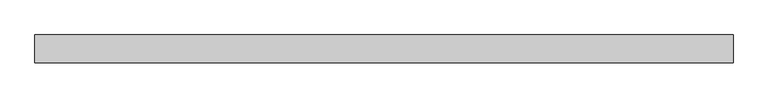
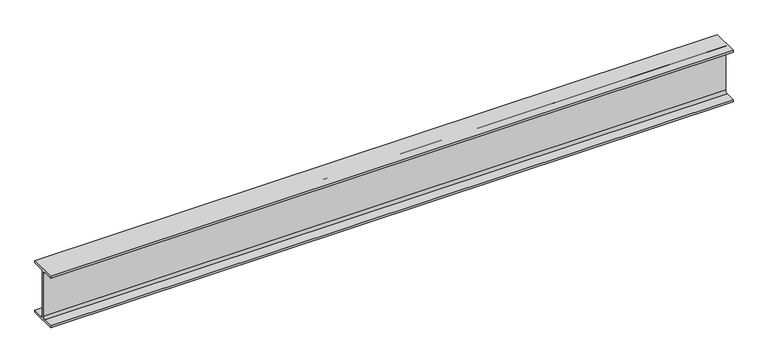
"""IFC4 building model written with IfcOpenShell, lengths in millimetres: beam geometry, 0912_Steel Framing_H-KSD3502 : H_SB_ASB_H-250x125x6x9."""

import ifcopenshell
import ifcopenshell.guid

model = None  # the IFC model being written
_history = None  # IfcOwnerHistory: only IFC2X3 demands one
_inside = {}  # id of a spatial element -> (the spatial element, [elements in it])
_under = {}  # id of a project, library or spatial element -> (it, [spatial elements below it])
_declared = {}  # id of a project -> (the project, [libraries it declares])
_typed = {}  # id of a type object -> (the type object, [elements of that type])
_made_of = {}  # id of a material, layer set ... -> (it, [elements and type objects made of it])


def new_model(schema):
    """Start an empty IFC model of exactly this schema.

    Asked for "IFC4X3", IfcOpenShell would pick the latest addendum, in which some entities
    have other attributes; the version numbers below select the first issue.
    IFC2X3 requires an IfcOwnerHistory on every rooted entity: one is made here for all.
    """
    global model, _history
    if schema == "IFC4X3":
        model = ifcopenshell.file(schema_version=(4, 3, 0, 0))
    else:
        model = ifcopenshell.file(schema=schema)
    _inside.clear()
    _under.clear()
    _declared.clear()
    _typed.clear()
    _made_of.clear()
    _history = None
    if model.schema == "IFC2X3":
        org = make("IfcOrganization", Name="unknown")
        user = make(
            "IfcPersonAndOrganization",
            ThePerson=make("IfcPerson", FamilyName="unknown"),
            TheOrganization=org,
        )
        app = make(
            "IfcApplication",
            ApplicationDeveloper=org,
            Version="unknown",
            ApplicationFullName="unknown",
            ApplicationIdentifier="unknown",
        )
        _history = make(
            "IfcOwnerHistory",
            OwningUser=user,
            OwningApplication=app,
            ChangeAction="ADDED",
            CreationDate=0,
        )
    return model


def make(cls, **values):
    """One entity of the class cls with the attributes given. An attribute that is None is left unset."""
    return model.create_entity(
        cls, **{name: value for name, value in values.items() if value is not None}
    )


def rooted(cls, **values):
    """An entity with a GlobalId (a new one), such as an element, a storey or a relation."""
    return make(cls, GlobalId=ifcopenshell.guid.new(), OwnerHistory=_history, **values)


def si_unit(unit_type, name, prefix=None):
    """IfcSIUnit, for example si_unit("LENGTHUNIT", "METRE", prefix="MILLI")."""
    return make("IfcSIUnit", UnitType=unit_type, Prefix=prefix, Name=name)


def assignment(units):
    """IfcUnitAssignment: the units of a project."""
    return None if units is None else make("IfcUnitAssignment", Units=units)


def point(xyz):
    """IfcCartesianPoint."""
    return None if xyz is None else make("IfcCartesianPoint", Coordinates=xyz)


def direction(xyz):
    """IfcDirection."""
    return None if xyz is None else make("IfcDirection", DirectionRatios=xyz)


def frame(location, z_axis=None, x_axis=None):
    """IfcAxis2Placement3D, a coordinate frame: its origin and axes. An axis left out is left unset."""
    return make(
        "IfcAxis2Placement3D",
        Location=point(location),
        Axis=direction(z_axis),
        RefDirection=direction(x_axis),
    )


def frame_2d(location, x_axis=None):
    """IfcAxis2Placement2D, a coordinate frame in the plane: its origin and x axis."""
    return make(
        "IfcAxis2Placement2D", Location=point(location), RefDirection=direction(x_axis)
    )


def origin():
    """The frame at (0, 0, 0) with its axes left unset."""
    return frame((0.0, 0.0, 0.0))


def place(relative_to, where):
    """IfcLocalPlacement: puts the frame where relative to a parent placement (None: the world)."""
    return make(
        "IfcLocalPlacement", PlacementRelTo=relative_to, RelativePlacement=where
    )


def context(
    kind, dimensions, precision=None, world=None, true_north=None, identifier=None
):
    """IfcGeometricRepresentationContext, for example the 3D "Model" context."""
    return make(
        "IfcGeometricRepresentationContext",
        ContextIdentifier=identifier,
        ContextType=kind,
        CoordinateSpaceDimension=dimensions,
        Precision=precision,
        WorldCoordinateSystem=world,
        TrueNorth=true_north,
    )


def project(units=None, contexts=None):
    """IfcProject with its units and contexts."""
    return rooted(
        "IfcProject",
        Name="project",
        RepresentationContexts=contexts,
        UnitsInContext=assignment(units),
    )


def spatial(cls, under=None, at=None, **own):
    """A site, building, storey or space (cls), placed at a placement, below another one or the project."""
    s = rooted(cls, ObjectPlacement=at, **own)
    if under is not None:
        _under.setdefault(under.id(), (under, []))[1].append(s)
    return s


def polyline(points):
    """IfcPolyline through the points."""
    return make("IfcPolyline", Points=[point(p) for p in points])


def circle_curve(where, radius):
    """IfcCircle in the frame where."""
    return make("IfcCircle", Position=where, Radius=radius)


def trimmed(basis, trim1, trim2, sense, master):
    """IfcTrimmedCurve: the piece of a basis curve between two trims."""
    return make(
        "IfcTrimmedCurve",
        BasisCurve=basis,
        Trim1=trim1,
        Trim2=trim2,
        SenseAgreement=sense,
        MasterRepresentation=master,
    )


def segment(curve, same_sense, transition):
    """IfcCompositeCurveSegment."""
    return make(
        "IfcCompositeCurveSegment",
        Transition=transition,
        SameSense=same_sense,
        ParentCurve=curve,
    )


def composite_curve(segments, self_intersect=None):
    """IfcCompositeCurve: segments joined end to end."""
    return make("IfcCompositeCurve", Segments=segments, SelfIntersect=self_intersect)


def outline(outer, holes=None, kind="AREA"):
    """IfcArbitraryClosedProfileDef: a profile drawn as a closed curve; with holes, ...WithVoids."""
    if holes is None:
        return make("IfcArbitraryClosedProfileDef", ProfileType=kind, OuterCurve=outer)
    return make(
        "IfcArbitraryProfileDefWithVoids",
        ProfileType=kind,
        OuterCurve=outer,
        InnerCurves=holes,
    )


def extrude(swept, where, along, depth):
    """IfcExtrudedAreaSolid: the profile swept, set in the frame where, extruded along a direction by depth."""
    return make(
        "IfcExtrudedAreaSolid",
        SweptArea=swept,
        Position=where,
        ExtrudedDirection=direction(along),
        Depth=depth,
    )


def shape(context_of_items, identifier, shape_type, items):
    """IfcShapeRepresentation: the items that make up one representation, for example the "Body"."""
    return make(
        "IfcShapeRepresentation",
        ContextOfItems=context_of_items,
        RepresentationIdentifier=identifier,
        RepresentationType=shape_type,
        Items=items,
    )


def source(mapping_origin, context_of_items, identifier, shape_type, items):
    """IfcRepresentationMap: a shape defined once, which mapped items show again and again."""
    return make(
        "IfcRepresentationMap",
        MappingOrigin=mapping_origin,
        MappedRepresentation=shape(context_of_items, identifier, shape_type, items),
    )


def transform(
    local_origin,
    x_axis=None,
    y_axis=None,
    z_axis=None,
    scale=None,
    scale2=None,
    scale3=None,
    uniform=True,
):
    """IfcCartesianTransformationOperator3D, or its non-uniform kind. x_axis, y_axis, z_axis: its Axis1, 2, 3."""
    if uniform:
        return make(
            "IfcCartesianTransformationOperator3D",
            Axis1=direction(x_axis),
            Axis2=direction(y_axis),
            LocalOrigin=point(local_origin),
            Scale=scale,
            Axis3=direction(z_axis),
        )
    return make(
        "IfcCartesianTransformationOperator3DnonUniform",
        Axis1=direction(x_axis),
        Axis2=direction(y_axis),
        LocalOrigin=point(local_origin),
        Scale=scale,
        Axis3=direction(z_axis),
        Scale2=scale2,
        Scale3=scale3,
    )


def mapped(mapping_source, mapping_target):
    """IfcMappedItem: shows the shape of a source again, moved by a transform."""
    return make(
        "IfcMappedItem", MappingSource=mapping_source, MappingTarget=mapping_target
    )


def made_of(thing, what):
    """Note that an element or type object is made of a material, layer set ...; save() writes the relation."""
    if what is not None:
        _made_of.setdefault(what.id(), (what, []))[1].append(thing)
    return thing


def element(
    cls,
    number,
    at=None,
    inside=None,
    cuts=None,
    type_object=None,
    material=None,
    context=None,
    identifier="Body",
    shape_type=None,
    held_by="IfcProductDefinitionShape",
    body=None,
    shapes=None,
    **own,
):
    """One element of the class cls, such as IfcWall. Its Tag is "e" and its number.

    at: its placement. inside: the storey or other place that contains it. cuts: it is an
    opening in that element (IfcRelVoidsElement). A single representation is given by context,
    identifier, shape_type and body (its items); several are given by shapes. held_by: the class
    of the entity that holds the representations. save() writes the other relations.
    """
    e = rooted(cls, Tag="e%d" % number, ObjectPlacement=at, **own)
    if body is not None:
        shapes = [shape(context, identifier, shape_type, body)]
    if shapes is not None:
        e.Representation = make(held_by, Representations=shapes)
    if inside is not None:
        _inside.setdefault(inside.id(), (inside, []))[1].append(e)
    if cuts is not None:
        rooted(
            "IfcRelVoidsElement", RelatingBuildingElement=cuts, RelatedOpeningElement=e
        )
    if type_object is not None:
        _typed.setdefault(type_object.id(), (type_object, []))[1].append(e)
    return made_of(e, material)


def aggregate(whole, parts):
    """IfcRelAggregates: a whole, such as a stair, and the parts it consists of."""
    return rooted("IfcRelAggregates", RelatingObject=whole, RelatedObjects=parts)


def save(model, path):
    """Write the relations noted so far, then the file.

    IfcRelAggregates (storeys below a building ...), IfcRelContainedInSpatialStructure (elements
    in a storey), IfcRelDefinesByType, IfcRelAssociatesMaterial and IfcRelDeclares: one each for
    every whole, place, type object, material and project.
    """
    for whole, parts in _under.values():
        aggregate(whole, parts)
    for where, things in _inside.values():
        rooted(
            "IfcRelContainedInSpatialStructure",
            RelatedElements=things,
            RelatingStructure=where,
        )
    for kind, things in _typed.values():
        rooted("IfcRelDefinesByType", RelatedObjects=things, RelatingType=kind)
    for what, things in _made_of.values():
        rooted("IfcRelAssociatesMaterial", RelatedObjects=things, RelatingMaterial=what)
    for by, libraries in _declared.values():
        rooted("IfcRelDeclares", RelatingContext=by, RelatedDefinitions=libraries)
    model.write(path)


def beam_d4d7e5cf(model_context):
    return source(origin(), model_context, "Body", "SweptSolid", [
        extrude(outline(composite_curve([segment(polyline([(62.5, -116.0), (62.5, -125.0), (-62.5, -125.0), (-62.5, -116.0), (-15.0, -116.0)]), True, "CONTINUOUS"), segment(trimmed(circle_curve(frame_2d((-15.0, -104.0)), 12.0), [point((-15.0, -116.0))], [point((-3.0, -104.0))], True, "CARTESIAN"), True, "CONTINUOUS"), segment(polyline([(-3.0, -104.0), (-3.0, 104.0)]), True, "CONTINUOUS"), segment(trimmed(circle_curve(frame_2d((-15.0, 104.0)), 12.0), [point((-3.0, 104.0))], [point((-15.0, 116.0))], True, "CARTESIAN"), True, "CONTINUOUS"), segment(polyline([(-15.0, 116.0), (-62.5, 116.0), (-62.5, 125.0), (62.5, 125.0), (62.5, 116.0), (15.0, 116.0)]), True, "CONTINUOUS"), segment(trimmed(circle_curve(frame_2d((15.0, 104.0)), 12.0), [point((15.0, 116.0))], [point((3.0, 104.0))], True, "CARTESIAN"), True, "CONTINUOUS"), segment(polyline([(3.0, 104.0), (3.0, -104.0)]), True, "CONTINUOUS"), segment(trimmed(circle_curve(frame_2d((15.0, -104.0)), 12.0), [point((3.0, -104.0))], [point((15.0, -116.0))], True, "CARTESIAN"), True, "CONTINUOUS"), segment(polyline([(15.0, -116.0), (62.5, -116.0)]), True, "CONTINUOUS")], self_intersect=False)), frame((-1494.4889476, 0.0, 0.0), z_axis=(1.0, 0.0, 0.0), x_axis=(0.0, 1.0, 0.0)), (0.0, 0.0, 1.0), 3149.288991),
    ])


if __name__ == "__main__":
    model = new_model("IFC4")
    model_context = context("Model", 3, world=origin())
    ifc_project = project(units=[si_unit("LENGTHUNIT", "METRE", prefix="MILLI")], contexts=[model_context])
    site = spatial("IfcSite", under=ifc_project)
    building = spatial("IfcBuilding", under=site)
    placement = place(None, origin())
    beam_shape = beam_d4d7e5cf(model_context)
    element("IfcBeam", 1, ObjectType="0912_Steel Framing_H-KSD3502 : H_SB_ASB_H-250x125x6x9", at=placement, inside=building, context=model_context, shape_type="MappedRepresentation", body=[
        mapped(beam_shape, transform((0.0, 0.0, 0.0), x_axis=(1.0, 0.0, 0.0), y_axis=(0.0, 1.0, 0.0), z_axis=(0.0, 0.0, 1.0))),
    ])
    save(model, "model.ifc")

# Revit data of these elements
# Type "0912_Steel Framing_H-KSD3502 : H_SB_ASB_H-250x125x6x9"
#   H_WM Code_1 = "S01AA003-00001 | Main Steel Structure Fabrication Work | Shelter/Building | Light Steel - Standard (30KG/M>Weight) | Material: (   )"
#   H_WM Code_2 = "S03AA029-00001 | Main Steel Structure Erection Work | Shelter/Building | Light Steel (30KG/M>Weight) | Material: (   )"
#   H_WM Code_3 = "S01AA010-00001 | Main Steel Structure Fabrication Work | Shelter/Building | Steel Painting/Coating | for Non-Fireproofed Steel Surface, Surface Preparation, Primer, Second & Final Coat | Material: (   )"
#   H_Q'ty Cal Type Tag = "SB-Q2"
#   Width = 12.5 cm
#   Web Thickness = 0.6 cm
#   Web Fillet = 1.2 cm
#   Warping Constant = 42539.8 cm⁶
#   W = 0
#   Torsional Moment of Inertia = 7.8102 cm⁴
#   Section Area = 37.66 cm²
#   Plastic Modulus weak axis = 73.1 cm³
#   Plastic Modulus strong axis = 366.0 cm³
#   Perimeter = 0.97 m²/m
#   Nominal Weight = 29.60 kgf/m
#   Moment of Inertia weak axis = 294.00 cm⁴
#   Moment of Inertia strong axis = 4050.00 cm⁴
#   Height = 25.0 cm
#   Flange Thickness = 0.9 cm
#   Elastic Modulus weak axis = 47.0 cm³
#   Elastic Modulus strong axis = 324.0 cm³
#   Centroid Vertical = 12.5 cm
#   Centroid Horizontal = 6.25 cm
#   Ix = 40500000
#   Length [instance default] = 1.5240 m
#   Zx = 366000
#   b = 0.1250 m
#   h = 0.2500 m
#   r = 0.0120 m
#   s = 0.0060 m
#   t = 0.0090 m
#   A = 0.003766 m²
#   Structural Material [instance default] = Steel, 45-345
#   Assembly Code = ""
# Element 1 (IfcBeam, "0912_Steel Framing_H-KSD3502 : H_SB_ASB_H-250x125x6x9")
#   Structural Material = none
# Materials
#   "Steel, 45-345": class "Metal", colour RGB 189 187 185, transparency 0, Description = "Steel 345 MPa", Cost = 0
